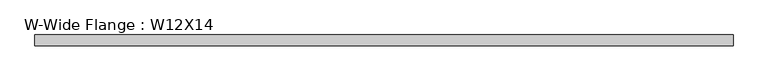
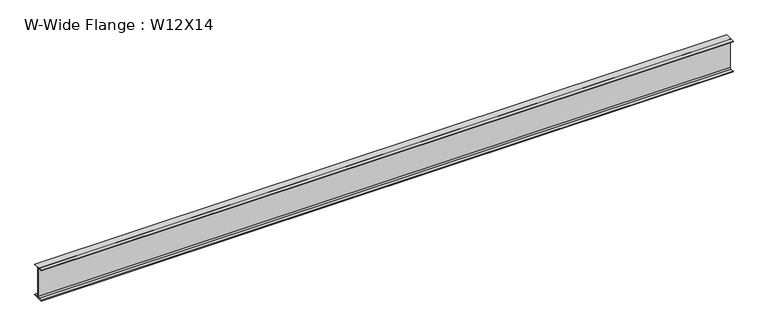
"""IFC4 building model written with IfcOpenShell, lengths in millimetres: beam geometry, W-Wide Flange : W12X14."""

from ifc_helpers import new_model, si_unit, point, frame, frame_2d, origin, place, context, project, spatial, polyline, circle_curve, trimmed, segment, composite_curve, outline, extrude, source, transform, mapped, element, save


def w_wide_flange_w12x14_635e0d45(model_context):
    return source(origin(), model_context, "Body", "SweptSolid", [
        extrude(outline(composite_curve([segment(polyline([(50.419, -145.415), (50.419, -151.13), (-50.419, -151.13), (-50.419, -145.415), (-15.875, -145.415)]), True, "CONTINUOUS"), segment(trimmed(circle_curve(frame_2d((-15.875, -132.08)), 13.335), [point((-15.875, -145.415))], [point((-2.54, -132.08))], True, "CARTESIAN"), True, "CONTINUOUS"), segment(polyline([(-2.54, -132.08), (-2.54, 132.08)]), True, "CONTINUOUS"), segment(trimmed(circle_curve(frame_2d((-15.875, 132.08)), 13.335), [point((-2.54, 132.08))], [point((-15.875, 145.415))], True, "CARTESIAN"), True, "CONTINUOUS"), segment(polyline([(-15.875, 145.415), (-50.419, 145.415), (-50.419, 151.13), (50.419, 151.13), (50.419, 145.415), (15.875, 145.415)]), True, "CONTINUOUS"), segment(trimmed(circle_curve(frame_2d((15.875, 132.08)), 13.335), [point((15.875, 145.415))], [point((2.54, 132.08))], True, "CARTESIAN"), True, "CONTINUOUS"), segment(polyline([(2.54, 132.08), (2.54, -132.08)]), True, "CONTINUOUS"), segment(trimmed(circle_curve(frame_2d((15.875, -132.08)), 13.335), [point((2.54, -132.08))], [point((15.875, -145.415))], True, "CARTESIAN"), True, "CONTINUOUS"), segment(polyline([(15.875, -145.415), (50.419, -145.415)]), True, "CONTINUOUS")], self_intersect=False)), frame((-3227.0938125, 0.0, 0.0), z_axis=(1.0, 0.0, 0.0), x_axis=(0.0, 1.0, 0.0)), (0.0, 0.0, 1.0), 6422.437625),
    ])


if __name__ == "__main__":
    model = new_model("IFC4")
    model_context = context("Model", 3, world=origin())
    ifc_project = project(units=[si_unit("LENGTHUNIT", "METRE", prefix="MILLI")], contexts=[model_context])
    site = spatial("IfcSite", under=ifc_project)
    building = spatial("IfcBuilding", under=site)
    placement = place(None, origin())
    w_wide_flange_w12x14_shape = w_wide_flange_w12x14_635e0d45(model_context)
    element("IfcBeam", 1, ObjectType="W-Wide Flange : W12X14", at=placement, inside=building, context=model_context, shape_type="MappedRepresentation", body=[
        mapped(w_wide_flange_w12x14_shape, transform((0.0, 0.0, 0.0), x_axis=(1.0, 0.0, 0.0), y_axis=(0.0, 1.0, 0.0), z_axis=(0.0, 0.0, 1.0))),
    ])
    save(model, "model.ifc")

# Revit data of these elements
# Type "W-Wide Flange : W12X14"
#   Assembly Code = "B10"
#   W = 14
#   Length [instance default] = 5' - 0"
#   bf = 0' - 3.97"
#   d = 0' - 11.9"
#   k = 0' - 0 3/4"
#   k2 = 0' - 0.525"
#   tf = 0' - 0.225"
#   tw = 0' - 0.2"
#   A = 0.0288889 SF
#   Structural Material [instance default] = Steel ASTM A992
# Element 1 (IfcBeam, "W-Wide Flange : W12X14")
#   Materials on its faces: "Steel ASTM A992"
# Materials
#   "Steel ASTM A992": class "Metal", colour RGB 199 199 199, transparency 0, Description = "Structural steel 50ksi", Cost = 0
